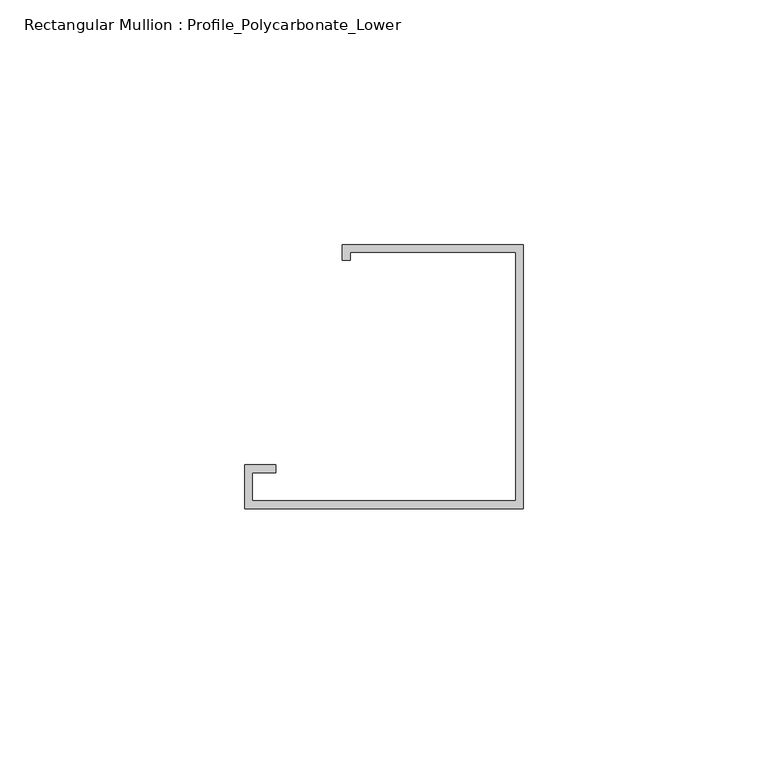
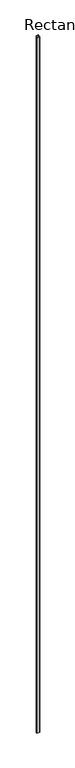
"""IFC4 building model written with IfcOpenShell, lengths in millimetres: member geometry, Rectangular Mullion : Profile_Polycarbonate_Lower."""

from ifc_helpers import new_model, si_unit, frame, origin, place, context, project, spatial, polyline, outline, extrude, source, transform, mapped, element, save


def rectangular_mullion_profile_polycarbonate_lower_911a9afa(model_context):
    return source(origin(), model_context, "Body", "SweptSolid", [
        extrude(outline(polyline([(0.0, -28.984575), (-56.9976, -28.984575), (-56.9976, -19.992975), (-50.6476, -19.992975), (-50.6476, -21.580475), (-55.4101, -21.580475), (-55.4101, -27.397075), (-1.5875, -27.397075), (-1.5875, 23.428325), (-35.3949, 23.428325), (-35.3949, 21.840825), (-36.9824, 21.840825), (-36.9824, 25.015825), (0.0, 25.015825), (0.0, -28.984575)])), frame((0.0, 0.0, -13290.7024), z_axis=(0.0, 0.0, 1.0), x_axis=(1.0, 0.0, 0.0)), (0.0, 0.0, 1.0), 13290.7024),
    ])


if __name__ == "__main__":
    model = new_model("IFC4")
    model_context = context("Model", 3, world=origin())
    ifc_project = project(units=[si_unit("LENGTHUNIT", "METRE", prefix="MILLI")], contexts=[model_context])
    site = spatial("IfcSite", under=ifc_project)
    building = spatial("IfcBuilding", under=site)
    placement = place(None, origin())
    rectangular_mullion_profile_polycarbonate_lower_shape = rectangular_mullion_profile_polycarbonate_lower_911a9afa(model_context)
    element("IfcMember", 1, ObjectType="Rectangular Mullion : Profile_Polycarbonate_Lower", at=placement, inside=building, context=model_context, shape_type="MappedRepresentation", body=[
        mapped(rectangular_mullion_profile_polycarbonate_lower_shape, transform((0.0, 0.0, 0.0), x_axis=(1.0, 0.0, 0.0), y_axis=(0.0, 1.0, 0.0), z_axis=(0.0, 0.0, 1.0))),
    ])
    save(model, "model.ifc")

# Revit data of these elements
# Type "Rectangular Mullion : Profile_Polycarbonate_Lower"
#   built-in parameter 1007322 = 0.177167 (stored number, unit not read)
#   built-in parameter 1007321 = 0 (stored number, unit not read)
#   built-in parameter 1007320 = 0.00520833 (stored number, unit not read)
